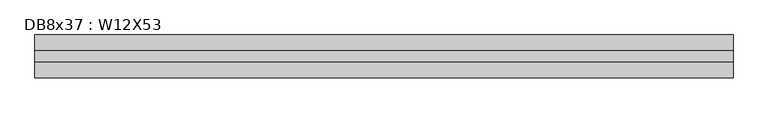
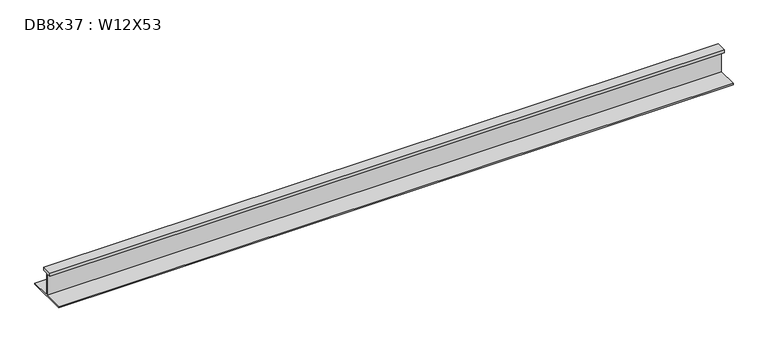
"""IFC4 building model written with IfcOpenShell, lengths in millimetres: beam geometry, DB8x37 : W12X53."""

from ifc_helpers import new_model, si_unit, frame, origin, place, context, project, spatial, polyline, outline, extrude, source, transform, mapped, element, save


def db8x37_w12x53_371747f4(model_context):
    return source(origin(), model_context, "Body", "SweptSolid", [
        extrude(outline(polyline([(38.1, 145.415), (38.1, 120.015), (2.921, 120.015), (2.921, -48.4505), (152.4, -48.4505), (152.4, -58.1025), (-152.4, -58.1025), (-152.4, -48.4505), (-2.921, -48.4505), (-2.921, 120.015), (-38.1, 120.015), (-38.1, 145.415), (38.1, 145.415)])), frame((-2490.216, 0.0, 0.0), z_axis=(1.0, 0.0, 0.0), x_axis=(0.0, 1.0, 0.0)), (0.0, 0.0, 1.0), 4982.845),
    ])


if __name__ == "__main__":
    model = new_model("IFC4")
    model_context = context("Model", 3, world=origin())
    ifc_project = project(units=[si_unit("LENGTHUNIT", "METRE", prefix="MILLI")], contexts=[model_context])
    site = spatial("IfcSite", under=ifc_project)
    building = spatial("IfcBuilding", under=site)
    placement = place(None, origin())
    db8x37_w12x53_shape = db8x37_w12x53_371747f4(model_context)
    element("IfcBeam", 1, ObjectType="DB8x37 : W12X53", at=placement, inside=building, context=model_context, shape_type="MappedRepresentation", body=[
        mapped(db8x37_w12x53_shape, transform((0.0, 0.0, 0.0), x_axis=(1.0, 0.0, 0.0), y_axis=(0.0, 1.0, 0.0), z_axis=(0.0, 0.0, 1.0))),
    ])
    save(model, "model.ifc")

# Revit data of these elements
# Type "DB8x37 : W12X53"
#   Assembly Code = "B10"
#   W = 53
#   Length [instance default] = 5' - 0"
#   bf = 0' - 10"
#   d = 1' - 0.1"
#   k = 0' - 1 3/8"
#   k2 = 0' - 0.8"
#   tf = 0' - 0.575"
#   tw = 0' - 0.345"
#   A = 0.108333 SF
#   Structural Material [instance default] = Steel ASTM A992
# Element 1 (IfcBeam, "DB8x37 : W12X53")
#   Materials on its faces: "Steel ASTM A992"
# Materials
#   "Steel ASTM A992": class "Metal", colour RGB 199 199 199, transparency 0, Description = "Structural steel 50ksi", Cost = 0
